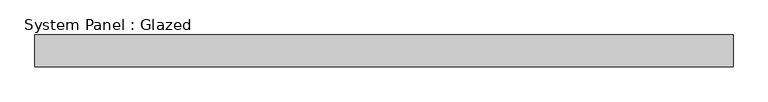
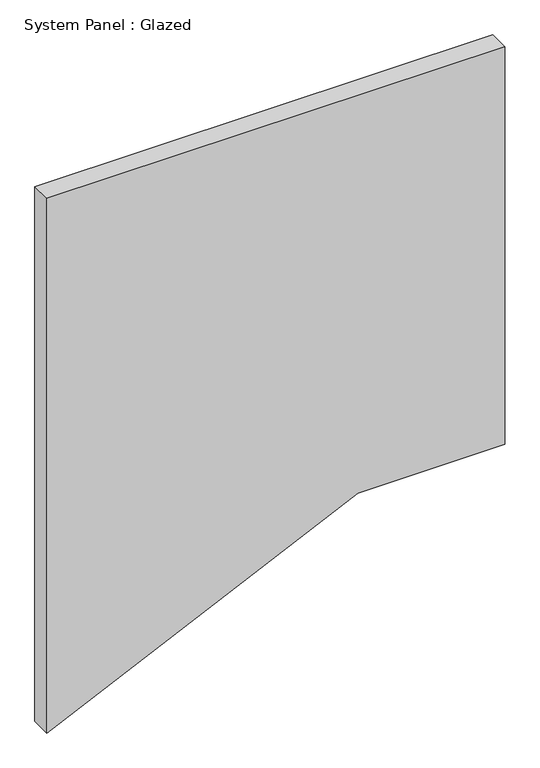
"""IFC4 building model written with IfcOpenShell, lengths in millimetres: plate geometry, System Panel : Glazed."""

from ifc_helpers import new_model, si_unit, frame, origin, place, context, project, spatial, polyline, outline, extrude, source, transform, mapped, element, save


def system_panel_glazed_fb8f064f(model_context):
    return source(origin(), model_context, "Body", "SweptSolid", [
        extrude(outline(polyline([(0.0, -550.0006382), (347.9562441, 196.1947247), (347.9562441, 550.0006382), (1357.9562441, 550.0006382), (1357.9562441, -550.0006382), (0.0, -550.0006382)])), frame((0.0, -25.0, 0.0), z_axis=(0.0, 1.0, 0.0), x_axis=(0.0, 0.0, 1.0)), (0.0, 0.0, 1.0), 50.0),
    ])


if __name__ == "__main__":
    model = new_model("IFC4")
    model_context = context("Model", 3, world=origin())
    ifc_project = project(units=[si_unit("LENGTHUNIT", "METRE", prefix="MILLI")], contexts=[model_context])
    site = spatial("IfcSite", under=ifc_project)
    building = spatial("IfcBuilding", under=site)
    placement = place(None, origin())
    system_panel_glazed_shape = system_panel_glazed_fb8f064f(model_context)
    element("IfcPlate", 1, ObjectType="System Panel : Glazed", at=placement, inside=building, context=model_context, shape_type="MappedRepresentation", body=[
        mapped(system_panel_glazed_shape, transform((0.0, 0.0, 0.0), x_axis=(1.0, 0.0, 0.0), y_axis=(0.0, 1.0, 0.0), z_axis=(0.0, 0.0, 1.0))),
    ])
    save(model, "model.ifc")

# Revit data of these elements
# Type "System Panel : Glazed"
#   Type Mark = "CW-GLASS"
# Element 1 (IfcPlate, "System Panel : Glazed")
#   Materials on its faces: "Glass_Clear"
# Materials
#   "Glass_Clear": class "Glass", colour RGB 128 128 255, transparency 0.8, Comments = "Rendering appearance not upgraded ", Cost = 0
